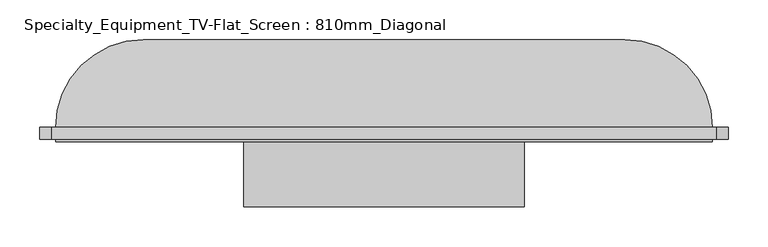
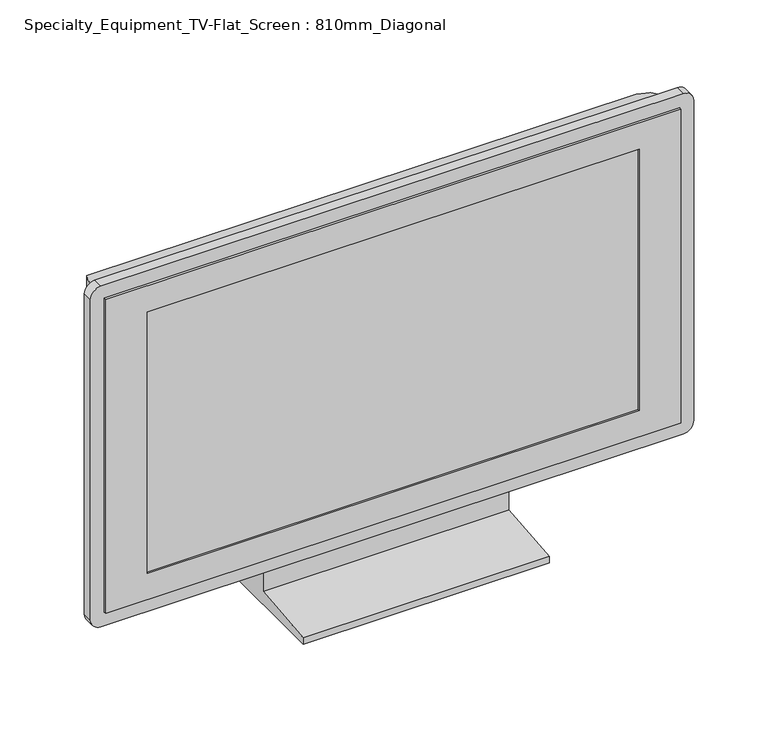
"""IFC4 building model written with IfcOpenShell, lengths in millimetres: proxy geometry, Specialty_Equipment_TV-Flat_Screen : 810mm_Diagonal."""

import ifcopenshell
import ifcopenshell.guid

model = None  # the IFC model being written
_history = None  # IfcOwnerHistory: only IFC2X3 demands one
_inside = {}  # id of a spatial element -> (the spatial element, [elements in it])
_under = {}  # id of a project, library or spatial element -> (it, [spatial elements below it])
_declared = {}  # id of a project -> (the project, [libraries it declares])
_typed = {}  # id of a type object -> (the type object, [elements of that type])
_made_of = {}  # id of a material, layer set ... -> (it, [elements and type objects made of it])


def new_model(schema):
    """Start an empty IFC model of exactly this schema.

    Asked for "IFC4X3", IfcOpenShell would pick the latest addendum, in which some entities
    have other attributes; the version numbers below select the first issue.
    IFC2X3 requires an IfcOwnerHistory on every rooted entity: one is made here for all.
    """
    global model, _history
    if schema == "IFC4X3":
        model = ifcopenshell.file(schema_version=(4, 3, 0, 0))
    else:
        model = ifcopenshell.file(schema=schema)
    _inside.clear()
    _under.clear()
    _declared.clear()
    _typed.clear()
    _made_of.clear()
    _history = None
    if model.schema == "IFC2X3":
        org = make("IfcOrganization", Name="unknown")
        user = make(
            "IfcPersonAndOrganization",
            ThePerson=make("IfcPerson", FamilyName="unknown"),
            TheOrganization=org,
        )
        app = make(
            "IfcApplication",
            ApplicationDeveloper=org,
            Version="unknown",
            ApplicationFullName="unknown",
            ApplicationIdentifier="unknown",
        )
        _history = make(
            "IfcOwnerHistory",
            OwningUser=user,
            OwningApplication=app,
            ChangeAction="ADDED",
            CreationDate=0,
        )
    return model


def make(cls, **values):
    """One entity of the class cls with the attributes given. An attribute that is None is left unset."""
    return model.create_entity(
        cls, **{name: value for name, value in values.items() if value is not None}
    )


def rooted(cls, **values):
    """An entity with a GlobalId (a new one), such as an element, a storey or a relation."""
    return make(cls, GlobalId=ifcopenshell.guid.new(), OwnerHistory=_history, **values)


def si_unit(unit_type, name, prefix=None):
    """IfcSIUnit, for example si_unit("LENGTHUNIT", "METRE", prefix="MILLI")."""
    return make("IfcSIUnit", UnitType=unit_type, Prefix=prefix, Name=name)


def assignment(units):
    """IfcUnitAssignment: the units of a project."""
    return None if units is None else make("IfcUnitAssignment", Units=units)


def point(xyz):
    """IfcCartesianPoint."""
    return None if xyz is None else make("IfcCartesianPoint", Coordinates=xyz)


def direction(xyz):
    """IfcDirection."""
    return None if xyz is None else make("IfcDirection", DirectionRatios=xyz)


def frame(location, z_axis=None, x_axis=None):
    """IfcAxis2Placement3D, a coordinate frame: its origin and axes. An axis left out is left unset."""
    return make(
        "IfcAxis2Placement3D",
        Location=point(location),
        Axis=direction(z_axis),
        RefDirection=direction(x_axis),
    )


def frame_2d(location, x_axis=None):
    """IfcAxis2Placement2D, a coordinate frame in the plane: its origin and x axis."""
    return make(
        "IfcAxis2Placement2D", Location=point(location), RefDirection=direction(x_axis)
    )


def origin():
    """The frame at (0, 0, 0) with its axes left unset."""
    return frame((0.0, 0.0, 0.0))


def place(relative_to, where):
    """IfcLocalPlacement: puts the frame where relative to a parent placement (None: the world)."""
    return make(
        "IfcLocalPlacement", PlacementRelTo=relative_to, RelativePlacement=where
    )


def context(
    kind, dimensions, precision=None, world=None, true_north=None, identifier=None
):
    """IfcGeometricRepresentationContext, for example the 3D "Model" context."""
    return make(
        "IfcGeometricRepresentationContext",
        ContextIdentifier=identifier,
        ContextType=kind,
        CoordinateSpaceDimension=dimensions,
        Precision=precision,
        WorldCoordinateSystem=world,
        TrueNorth=true_north,
    )


def project(units=None, contexts=None):
    """IfcProject with its units and contexts."""
    return rooted(
        "IfcProject",
        Name="project",
        RepresentationContexts=contexts,
        UnitsInContext=assignment(units),
    )


def spatial(cls, under=None, at=None, **own):
    """A site, building, storey or space (cls), placed at a placement, below another one or the project."""
    s = rooted(cls, ObjectPlacement=at, **own)
    if under is not None:
        _under.setdefault(under.id(), (under, []))[1].append(s)
    return s


def polyline(points):
    """IfcPolyline through the points."""
    return make("IfcPolyline", Points=[point(p) for p in points])


def circle_curve(where, radius):
    """IfcCircle in the frame where."""
    return make("IfcCircle", Position=where, Radius=radius)


def ellipse_curve(where, semi_axis1, semi_axis2):
    """IfcEllipse in the frame where."""
    return make(
        "IfcEllipse", Position=where, SemiAxis1=semi_axis1, SemiAxis2=semi_axis2
    )


def trimmed(basis, trim1, trim2, sense, master):
    """IfcTrimmedCurve: the piece of a basis curve between two trims."""
    return make(
        "IfcTrimmedCurve",
        BasisCurve=basis,
        Trim1=trim1,
        Trim2=trim2,
        SenseAgreement=sense,
        MasterRepresentation=master,
    )


def segment(curve, same_sense, transition):
    """IfcCompositeCurveSegment."""
    return make(
        "IfcCompositeCurveSegment",
        Transition=transition,
        SameSense=same_sense,
        ParentCurve=curve,
    )


def composite_curve(segments, self_intersect=None):
    """IfcCompositeCurve: segments joined end to end."""
    return make("IfcCompositeCurve", Segments=segments, SelfIntersect=self_intersect)


def outline(outer, holes=None, kind="AREA"):
    """IfcArbitraryClosedProfileDef: a profile drawn as a closed curve; with holes, ...WithVoids."""
    if holes is None:
        return make("IfcArbitraryClosedProfileDef", ProfileType=kind, OuterCurve=outer)
    return make(
        "IfcArbitraryProfileDefWithVoids",
        ProfileType=kind,
        OuterCurve=outer,
        InnerCurves=holes,
    )


def extrude(swept, where, along, depth):
    """IfcExtrudedAreaSolid: the profile swept, set in the frame where, extruded along a direction by depth."""
    return make(
        "IfcExtrudedAreaSolid",
        SweptArea=swept,
        Position=where,
        ExtrudedDirection=direction(along),
        Depth=depth,
    )


def faces_of(points, faces, orient=None, outer=None):
    """IfcFace entities. A face is a list of loops; a loop is a list of indices into points, from 0.

    orient and outer hold one flag for each loop. By default every Orientation is true, the
    first loop of a face is its IfcFaceOuterBound and the others are IfcFaceBound.
    """
    made = []
    for i, loops in enumerate(faces):
        bounds = []
        for j, loop in enumerate(loops):
            is_outer = j == 0 if outer is None else outer[i][j]
            bounds.append(
                make(
                    "IfcFaceOuterBound" if is_outer else "IfcFaceBound",
                    Bound=make("IfcPolyLoop", Polygon=[points[k] for k in loop]),
                    Orientation=True if orient is None else orient[i][j],
                )
            )
        made.append(make("IfcFace", Bounds=bounds))
    return made


def faceted_brep(points, faces, orient=None, outer=None, voids=None):
    """IfcFacetedBrep: a solid bounded by flat faces; with voids (closed shells), ...WithVoids."""
    shared = [point(p) for p in points]
    hull = make("IfcClosedShell", CfsFaces=faces_of(shared, faces, orient, outer))
    if voids is None:
        return make("IfcFacetedBrep", Outer=hull)
    return make(
        "IfcFacetedBrepWithVoids",
        Outer=hull,
        Voids=[
            make(cls, CfsFaces=faces_of(shared, fs, o, b)) for cls, fs, o, b in voids
        ],
    )


def shape(context_of_items, identifier, shape_type, items):
    """IfcShapeRepresentation: the items that make up one representation, for example the "Body"."""
    return make(
        "IfcShapeRepresentation",
        ContextOfItems=context_of_items,
        RepresentationIdentifier=identifier,
        RepresentationType=shape_type,
        Items=items,
    )


def source(mapping_origin, context_of_items, identifier, shape_type, items):
    """IfcRepresentationMap: a shape defined once, which mapped items show again and again."""
    return make(
        "IfcRepresentationMap",
        MappingOrigin=mapping_origin,
        MappedRepresentation=shape(context_of_items, identifier, shape_type, items),
    )


def transform(
    local_origin,
    x_axis=None,
    y_axis=None,
    z_axis=None,
    scale=None,
    scale2=None,
    scale3=None,
    uniform=True,
):
    """IfcCartesianTransformationOperator3D, or its non-uniform kind. x_axis, y_axis, z_axis: its Axis1, 2, 3."""
    if uniform:
        return make(
            "IfcCartesianTransformationOperator3D",
            Axis1=direction(x_axis),
            Axis2=direction(y_axis),
            LocalOrigin=point(local_origin),
            Scale=scale,
            Axis3=direction(z_axis),
        )
    return make(
        "IfcCartesianTransformationOperator3DnonUniform",
        Axis1=direction(x_axis),
        Axis2=direction(y_axis),
        LocalOrigin=point(local_origin),
        Scale=scale,
        Axis3=direction(z_axis),
        Scale2=scale2,
        Scale3=scale3,
    )


def mapped(mapping_source, mapping_target):
    """IfcMappedItem: shows the shape of a source again, moved by a transform."""
    return make(
        "IfcMappedItem", MappingSource=mapping_source, MappingTarget=mapping_target
    )


def made_of(thing, what):
    """Note that an element or type object is made of a material, layer set ...; save() writes the relation."""
    if what is not None:
        _made_of.setdefault(what.id(), (what, []))[1].append(thing)
    return thing


def element(
    cls,
    number,
    at=None,
    inside=None,
    cuts=None,
    type_object=None,
    material=None,
    context=None,
    identifier="Body",
    shape_type=None,
    held_by="IfcProductDefinitionShape",
    body=None,
    shapes=None,
    **own,
):
    """One element of the class cls, such as IfcWall. Its Tag is "e" and its number.

    at: its placement. inside: the storey or other place that contains it. cuts: it is an
    opening in that element (IfcRelVoidsElement). A single representation is given by context,
    identifier, shape_type and body (its items); several are given by shapes. held_by: the class
    of the entity that holds the representations. save() writes the other relations.
    """
    e = rooted(cls, Tag="e%d" % number, ObjectPlacement=at, **own)
    if body is not None:
        shapes = [shape(context, identifier, shape_type, body)]
    if shapes is not None:
        e.Representation = make(held_by, Representations=shapes)
    if inside is not None:
        _inside.setdefault(inside.id(), (inside, []))[1].append(e)
    if cuts is not None:
        rooted(
            "IfcRelVoidsElement", RelatingBuildingElement=cuts, RelatedOpeningElement=e
        )
    if type_object is not None:
        _typed.setdefault(type_object.id(), (type_object, []))[1].append(e)
    return made_of(e, material)


def aggregate(whole, parts):
    """IfcRelAggregates: a whole, such as a stair, and the parts it consists of."""
    return rooted("IfcRelAggregates", RelatingObject=whole, RelatedObjects=parts)


def save(model, path):
    """Write the relations noted so far, then the file.

    IfcRelAggregates (storeys below a building ...), IfcRelContainedInSpatialStructure (elements
    in a storey), IfcRelDefinesByType, IfcRelAssociatesMaterial and IfcRelDeclares: one each for
    every whole, place, type object, material and project.
    """
    for whole, parts in _under.values():
        aggregate(whole, parts)
    for where, things in _inside.values():
        rooted(
            "IfcRelContainedInSpatialStructure",
            RelatedElements=things,
            RelatingStructure=where,
        )
    for kind, things in _typed.values():
        rooted("IfcRelDefinesByType", RelatedObjects=things, RelatingType=kind)
    for what, things in _made_of.values():
        rooted("IfcRelAssociatesMaterial", RelatedObjects=things, RelatingMaterial=what)
    for by, libraries in _declared.values():
        rooted("IfcRelDeclares", RelatingContext=by, RelatedDefinitions=libraries)
    model.write(path)


def plane_surface(at):
    """IfcPlane: the flat surface through the origin of the frame at, square to its z axis."""
    return make("IfcPlane", Position=at)


def cylinder_surface(at, radius):
    """IfcCylindricalSurface: all points at the distance radius from the z axis of the frame at."""
    return make("IfcCylindricalSurface", Position=at, Radius=radius)


def advanced_brep(points, edges, surfaces, faces):
    """IfcAdvancedBrep: a solid bounded by faces that lie on surfaces and meet in shared edges.

    An edge is (start, end): straight between two places in points (the first is 0);
    or (start, end, curve); or (start, end, curve, False) where it runs against its curve.
    A face is (place in surfaces, loops), or (place, loops, False) where it looks against
    its surface's normal. A loop lists edges by number (the first is 1), with a minus sign
    where the edge is run from its end to its start. The first loop is the outer one.
    """
    corners = [point(p) for p in points]
    vertices = [make("IfcVertexPoint", VertexGeometry=c) for c in corners]
    made = []
    for start, end, *more in edges:
        made.append(
            make(
                "IfcEdgeCurve",
                EdgeStart=vertices[start],
                EdgeEnd=vertices[end],
                EdgeGeometry=more[0] if more else make("IfcPolyline", Points=[corners[start], corners[end]]),
                SameSense=more[1] if len(more) > 1 else True,
            )
        )
    hull = []
    for where, loops, *sense in faces:
        bounds = []
        for j, loop in enumerate(loops):
            ring = [make("IfcOrientedEdge", EdgeElement=made[abs(k) - 1], Orientation=k > 0) for k in loop]
            bounds.append(
                make(
                    "IfcFaceOuterBound" if j == 0 else "IfcFaceBound",
                    Bound=make("IfcEdgeLoop", EdgeList=ring),
                    Orientation=True,
                )
            )
        hull.append(make("IfcAdvancedFace", Bounds=bounds, FaceSurface=surfaces[where], SameSense=sense[0] if sense else True))
    return make("IfcAdvancedBrep", Outer=make("IfcClosedShell", CfsFaces=hull))


def specialty_equipment_tv_flat_screen_810mm_diagonal_56245f3a(model_context):
    return source(origin(), model_context, "Body", "SolidModel", [
        extrude(outline(polyline([(-51.4613764, 80.0), (-1.4613764, 80.0), (48.5386236, 0.0), (-151.4613764, 0.0), (-151.4613764, 10.0), (-51.4613764, 20.0), (-51.4613764, 80.0)])), frame((-180.4346678, 0.0, 0.0), z_axis=(1.0, 0.0, 0.0), x_axis=(0.0, 1.0, 0.0)), (0.0, 0.0, 1.0), 352.9803073),
        faceted_brep([(409.0357931, -69.4613764, 557.1392838), (-416.9248214, -69.4613764, 557.1392838), (-416.9248214, -69.4613764, 80.0), (409.0357931, -69.4613764, 80.0), (-356.9248214, -69.4613764, 517.1392838), (349.0357931, -69.4613764, 517.1392838), (349.0357931, -69.4613764, 120.0), (-356.9248214, -69.4613764, 120.0), (409.0357931, -51.4613764, 557.1392838), (409.0357931, -51.4613764, 80.0), (-416.9248214, -51.4613764, 80.0), (-416.9248214, -51.4613764, 557.1392838), (-356.9248214, -66.4613764, 517.1392838), (-356.9248214, -66.4613764, 120.0), (349.0357931, -66.4613764, 120.0), (349.0357931, -66.4613764, 517.1392838)], [[[0, 1, 2, 3], [4, 5, 6, 7]], [[8, 9, 10, 11]], [[1, 0, 8, 11]], [[2, 1, 11, 10]], [[3, 2, 10, 9]], [[0, 3, 9, 8]], [[12, 13, 14, 15]], [[12, 15, 5, 4]], [[15, 14, 6, 5]], [[14, 13, 7, 6]], [[13, 12, 4, 7]]]),
        extrude(outline(composite_curve([segment(polyline([(577.1392838, 414.0357931), (577.1392838, -421.9248214)]), True, "CONTINUOUS"), segment(trimmed(circle_curve(frame_2d((562.1392838, -421.9248214)), 15.0), [point((577.1392838, -421.9248214))], [point((562.1392838, -436.9248214))], False, "CARTESIAN"), True, "CONTINUOUS"), segment(polyline([(562.1392838, -436.9248214), (75.0, -436.9248214)]), True, "CONTINUOUS"), segment(trimmed(circle_curve(frame_2d((75.0, -421.9248214)), 15.0), [point((75.0, -436.9248214))], [point((60.0, -421.9248214))], False, "CARTESIAN"), True, "CONTINUOUS"), segment(polyline([(60.0, -421.9248214), (60.0, 414.0357931)]), True, "CONTINUOUS"), segment(trimmed(circle_curve(frame_2d((75.0, 414.0357931)), 15.0), [point((60.0, 414.0357931))], [point((75.0, 429.0357931))], False, "CARTESIAN"), True, "CONTINUOUS"), segment(polyline([(75.0, 429.0357931), (562.1392838, 429.0357931)]), True, "CONTINUOUS"), segment(trimmed(circle_curve(frame_2d((562.1392838, 414.0357931)), 15.0), [point((562.1392838, 429.0357931))], [point((577.1392838, 414.0357931))], False, "CARTESIAN"), True, "CONTINUOUS")], self_intersect=False), holes=[polyline([(557.1392838, 409.0357931), (80.0, 409.0357931), (80.0, -416.9248214), (557.1392838, -416.9248214), (557.1392838, 409.0357931)])]), frame((0.0, -66.4613764, 0.0), z_axis=(0.0, 1.0, 0.0), x_axis=(0.0, 0.0, 1.0)), (0.0, 0.0, 1.0), 15.0),
        advanced_brep(
        [(-416.9248214, -51.4613764, 80.0), (409.0357931, -51.4613764, 80.0), (409.0357931, -51.4613764, 557.1392838), (-416.9248214, -51.4613764, 557.1392838), (299.0357931, 58.5386236, 80.0), (-306.9248214, 58.5386236, 80.0), (-306.9248214, 58.5386236, 447.1392838), (299.0357931, 58.5386236, 447.1392838)],
        [
            (0, 1),
            (1, 2),
            (2, 3),
            (3, 0),
            (4, 5),
            (5, 6),
            (6, 7),
            (7, 4),
            (0, 5, circle_curve(frame((-306.9248214, -51.4613764, 80.0), z_axis=(0.0, 0.0, -1.0), x_axis=(-1.0, 0.0, 0.0)), 110.0)),
            (4, 1, circle_curve(frame((299.0357931, -51.4613764, 80.0), z_axis=(0.0, 0.0, -1.0), x_axis=(1.0, 0.0, 0.0)), 110.0)),
            (7, 2, ellipse_curve(frame((299.0357931, -51.4613764, 447.1392838), z_axis=(0.7071067811865475, 0.0, -0.7071067811865475), x_axis=(0.7071067811865474, 0.0, 0.7071067811865476)), 155.5634919, 110.0)),
            (6, 3, ellipse_curve(frame((-306.9248214, -51.4613764, 447.1392838), z_axis=(0.7071067811865475, 0.0, 0.7071067811865475), x_axis=(-0.7071067811865476, 0.0, 0.7071067811865474)), 155.5634919, 110.0)),
        ],
        [
            plane_surface(frame((-416.9248214, -51.4613764, 557.1392838), z_axis=(0.0, -1.0, 0.0), x_axis=(-1.0, 0.0, 0.0))),
            plane_surface(frame((-416.9248214, 58.5386236, 557.1392838), z_axis=(0.0, 1.0, 0.0), x_axis=(1.0, 0.0, 0.0))),
            plane_surface(frame((-416.9248214, -51.4613764, 80.0), z_axis=(0.0, 0.0, -1.0), x_axis=(0.0, 1.0, 0.0))),
            cylinder_surface(frame((299.0357931, -51.4613764, 80.0), z_axis=(0.0, 0.0, 1.0), x_axis=(1.0, 0.0, 0.0)), 110.0),
            cylinder_surface(frame((409.0357931, -51.4613764, 447.1392838), z_axis=(-1.0, 0.0, 0.0), x_axis=(0.0, 0.0, 1.0)), 110.0),
            cylinder_surface(frame((-306.9248214, -51.4613764, 557.1392838), z_axis=(0.0, 0.0, -1.0), x_axis=(-1.0, 0.0, 0.0)), 110.0),
        ],
        [
            (0, [[1, 2, 3, 4]]),
            (1, [[5, 6, 7, 8]]),
            (2, [[-1, 9, -5, 10]]),
            (3, [[11, -2, -10, -8]]),
            (4, [[-11, -7, 12, -3]]),
            (5, [[-12, -6, -9, -4]]),
        ],
    ),
    ])


if __name__ == "__main__":
    model = new_model("IFC4")
    model_context = context("Model", 3, world=origin())
    ifc_project = project(units=[si_unit("LENGTHUNIT", "METRE", prefix="MILLI")], contexts=[model_context])
    site = spatial("IfcSite", under=ifc_project)
    building = spatial("IfcBuilding", under=site)
    placement = place(None, origin())
    specialty_equipment_tv_flat_screen_810mm_diagonal_shape = specialty_equipment_tv_flat_screen_810mm_diagonal_56245f3a(model_context)
    element("IfcBuildingElementProxy", 1, Name="Specialty_Equipment_TV-Flat_Screen : 810mm_Diagonal", ObjectType="Specialty_Equipment_TV-Flat_Screen : 810mm_Diagonal", at=placement, inside=building, context=model_context, shape_type="MappedRepresentation", body=[
        mapped(specialty_equipment_tv_flat_screen_810mm_diagonal_shape, transform((0.0, 0.0, 0.0), x_axis=(1.0, 0.0, 0.0), y_axis=(0.0, 1.0, 0.0), z_axis=(0.0, 0.0, 1.0))),
    ])
    save(model, "model.ifc")

# Revit data of these elements
# Type "Specialty_Equipment_TV-Flat_Screen : 810mm_Diagonal"
#   SinAng = 0.49 mm
#   L = 705.961 mm
#   H = 397.139 mm
#   Thickness = 110 mm
#   Diagonal = 810 mm
#   CosAng = 0.872 mm
#   Stand [instance default] = yes
#   Default Elevation = 0
# Element 1 (IfcBuildingElementProxy, "Specialty_Equipment_TV-Flat_Screen : 810mm_Diagonal")
#   Materials on its faces: "TV - Black", "TV - Glass", "TV - Screen"
# Materials
#   "TV - Black": class "Miscellaneous", colour RGB 49 49 49, transparency 0
#   "TV - Glass": class "Miscellaneous", colour RGB 157 157 157, transparency 0.9
#   "TV - Screen": class "Miscellaneous", colour RGB 0 0 0, transparency 0
